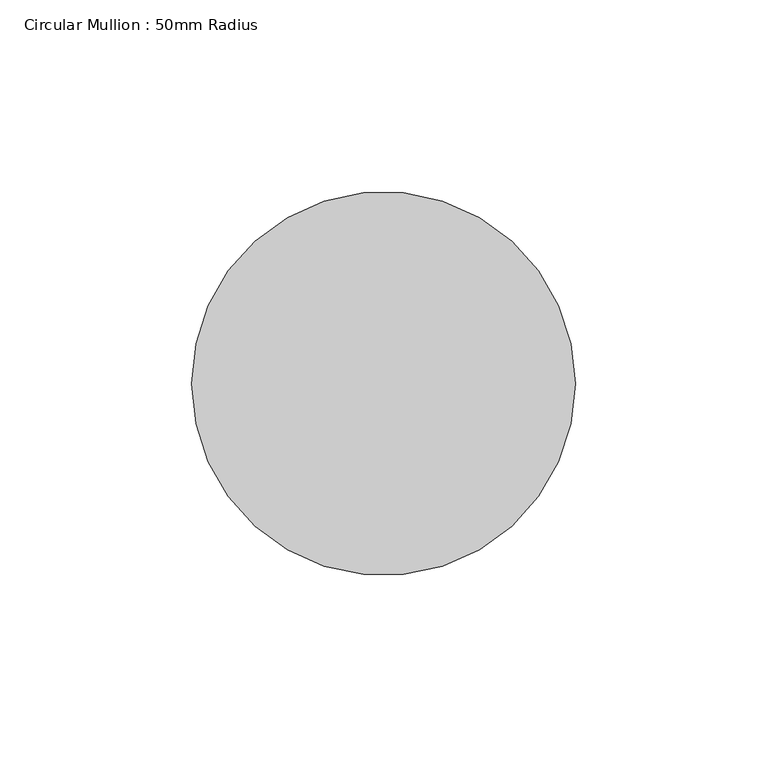
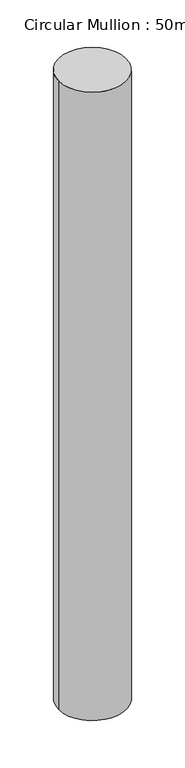
"""IFC4 building model written with IfcOpenShell, lengths in millimetres: member geometry, Circular Mullion : 50mm Radius."""

from ifc_helpers import new_model, si_unit, point, frame, origin, origin_2d, place, context, project, spatial, circle_curve, trimmed, segment, composite_curve, outline, extrude, source, transform, mapped, element, save


def circular_mullion_50mm_radius_32c08766(model_context):
    return source(origin(), model_context, "Body", "SweptSolid", [
        extrude(outline(composite_curve([segment(trimmed(circle_curve(origin_2d(), 50.0), [point((50.0, 0.0))], [point((-50.0, 0.0))], False, "CARTESIAN"), True, "CONTINUOUS"), segment(trimmed(circle_curve(origin_2d(), 50.0), [point((-50.0, 0.0))], [point((50.0, 0.0))], False, "CARTESIAN"), True, "CONTINUOUS")], self_intersect=False)), frame((0.0, 0.0, -980.6803632), z_axis=(0.0, 0.0, 1.0), x_axis=(1.0, 0.0, 0.0)), (0.0, 0.0, 1.0), 980.6803632),
    ])


if __name__ == "__main__":
    model = new_model("IFC4")
    model_context = context("Model", 3, world=origin())
    ifc_project = project(units=[si_unit("LENGTHUNIT", "METRE", prefix="MILLI")], contexts=[model_context])
    site = spatial("IfcSite", under=ifc_project)
    building = spatial("IfcBuilding", under=site)
    placement = place(None, origin())
    circular_mullion_50mm_radius_shape = circular_mullion_50mm_radius_32c08766(model_context)
    element("IfcMember", 1, ObjectType="Circular Mullion : 50mm Radius", at=placement, inside=building, context=model_context, shape_type="MappedRepresentation", body=[
        mapped(circular_mullion_50mm_radius_shape, transform((0.0, 0.0, 0.0), x_axis=(1.0, 0.0, 0.0), y_axis=(0.0, 1.0, 0.0), z_axis=(0.0, 0.0, 1.0))),
    ])
    save(model, "model.ifc")

# Revit data of these elements
# Type "Circular Mullion : 50mm Radius"
#   built-in parameter 1007350 = 0.164042 (stored number, unit not read)
# Element 1 (IfcMember, "Circular Mullion : 50mm Radius")
#   Materials on its faces: "Aluminium"
# Materials
#   "Aluminium": class "Metal", colour RGB 247 247 247, transparency 0, Description = "Aluminium 6061", Cost = 0
